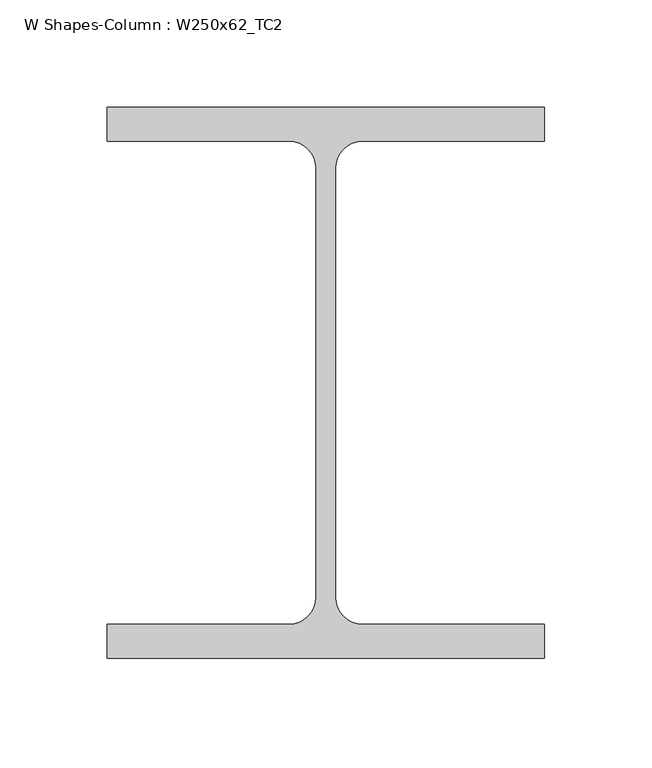
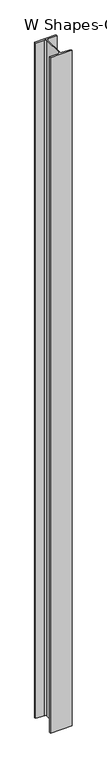
"""IFC4 building model written with IfcOpenShell, lengths in millimetres: column geometry, W Shapes-Column : W250x62_TC2."""

from ifc_helpers import new_model, si_unit, point, frame, frame_2d, origin, place, context, project, spatial, polyline, circle_curve, trimmed, segment, composite_curve, outline, extrude, source, transform, mapped, element, save


def w_shapes_column_w250x62_tc2_9f98f3c0(model_context):
    return source(origin(), model_context, "Body", "SweptSolid", [
        extrude(outline(composite_curve([segment(polyline([(101.854, 128.27), (101.854, 112.522), (17.145, 112.522)]), True, "CONTINUOUS"), segment(trimmed(circle_curve(frame_2d((17.145, 99.822)), 12.7), [point((17.145, 112.522))], [point((4.445, 99.822))], True, "CARTESIAN"), True, "CONTINUOUS"), segment(polyline([(4.445, 99.822), (4.445, -99.822)]), True, "CONTINUOUS"), segment(trimmed(circle_curve(frame_2d((17.145, -99.822)), 12.7), [point((4.445, -99.822))], [point((17.145, -112.522))], True, "CARTESIAN"), True, "CONTINUOUS"), segment(polyline([(17.145, -112.522), (101.854, -112.522), (101.854, -128.27), (-101.854, -128.27), (-101.854, -112.522), (-17.145, -112.522)]), True, "CONTINUOUS"), segment(trimmed(circle_curve(frame_2d((-17.145, -99.822)), 12.7), [point((-17.145, -112.522))], [point((-4.445, -99.822))], True, "CARTESIAN"), True, "CONTINUOUS"), segment(polyline([(-4.445, -99.822), (-4.445, 99.822)]), True, "CONTINUOUS"), segment(trimmed(circle_curve(frame_2d((-17.145, 99.822)), 12.7), [point((-4.445, 99.822))], [point((-17.145, 112.522))], True, "CARTESIAN"), True, "CONTINUOUS"), segment(polyline([(-17.145, 112.522), (-101.854, 112.522), (-101.854, 128.27), (101.854, 128.27)]), True, "CONTINUOUS")], self_intersect=False)), frame((0.0, 0.0, 200.0), z_axis=(0.0, 0.0, 1.0), x_axis=(1.0, 0.0, 0.0)), (0.0, 0.0, 1.0), 6750.0),
    ])


if __name__ == "__main__":
    model = new_model("IFC4")
    model_context = context("Model", 3, world=origin())
    ifc_project = project(units=[si_unit("LENGTHUNIT", "METRE", prefix="MILLI")], contexts=[model_context])
    site = spatial("IfcSite", under=ifc_project)
    building = spatial("IfcBuilding", under=site)
    placement = place(None, origin())
    w_shapes_column_w250x62_tc2_shape = w_shapes_column_w250x62_tc2_9f98f3c0(model_context)
    element("IfcColumn", 1, ObjectType="W Shapes-Column : W250x62_TC2", at=placement, inside=building, context=model_context, shape_type="MappedRepresentation", body=[
        mapped(w_shapes_column_w250x62_tc2_shape, transform((0.0, 0.0, 0.0), x_axis=(1.0, 0.0, 0.0), y_axis=(0.0, 1.0, 0.0), z_axis=(0.0, 0.0, 1.0))),
    ])
    save(model, "model.ifc")

# Revit data of these elements
# Type "W Shapes-Column : W250x62_TC2"
#   Section Name Key = "W10X45"
#   Assembly Code = "B10"
#   Width = 20.3708 cm
#   Web Thickness = 0.889 cm
#   Web Fillet = 1.27 cm
#   Warping Constant = 322243.0 cm⁶
#   Torsional Moment of Inertia = 62.8509 cm⁴
#   Section Area = 85.8063 cm²
#   Plastic Modulus weak axis = 332.657 cm³
#   Plastic Modulus strong axis = 899.65 cm³
#   Perimeter = 1.28778 m²/m
#   Nominal Weight = 66.9674 kgf/m
#   Moment of Inertia weak axis = 2222.68 cm⁴
#   Moment of Inertia strong axis = 10322.54 cm⁴
#   Height = 25.654 cm
#   Flange Thickness = 1.5748 cm
#   Elastic Modulus weak axis = 217.948 cm³
#   Elastic Modulus strong axis = 804.605 cm³
#   Clear Web Height = 19.05 cm
#   Centroid Vertical = 12.827 cm
#   Centroid Horizontal = 10.1854 cm
#   Bolt Spacing = 13.97 cm
#   Structural Material [instance default] = Steel ASTM A992
#   Principal Axes Angle = 0
# Element 1 (IfcColumn, "W Shapes-Column : W250x62_TC2")
#   Structural Material = none
# Materials
#   "Steel ASTM A992": class "Metal", colour RGB 199 199 199, transparency 0, Description = "Structural steel 50ksi", Cost = 0
